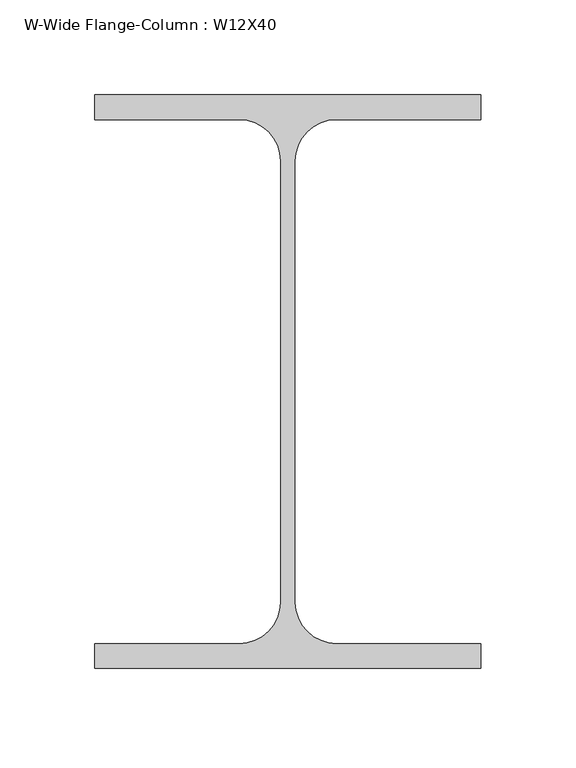
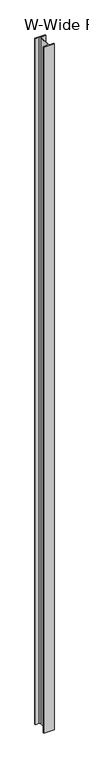
"""IFC4 building model written with IfcOpenShell, lengths in millimetres: column geometry, W-Wide Flange-Column : W12X40."""

from ifc_helpers import new_model, si_unit, point, frame, frame_2d, origin, place, context, project, spatial, polyline, circle_curve, trimmed, segment, composite_curve, outline, extrude, source, transform, mapped, element, save


def w_wide_flange_column_w12x40_26afb3f0(model_context):
    return source(origin(), model_context, "Body", "SweptSolid", [
        extrude(outline(composite_curve([segment(polyline([(101.727, 151.13), (101.727, 138.049), (25.5905, 138.049)]), True, "CONTINUOUS"), segment(trimmed(circle_curve(frame_2d((25.5905, 116.205)), 21.844), [point((25.5905, 138.049))], [point((3.7465, 116.205))], True, "CARTESIAN"), True, "CONTINUOUS"), segment(polyline([(3.7465, 116.205), (3.7465, -116.205)]), True, "CONTINUOUS"), segment(trimmed(circle_curve(frame_2d((25.5905, -116.205)), 21.844), [point((3.7465, -116.205))], [point((25.5905, -138.049))], True, "CARTESIAN"), True, "CONTINUOUS"), segment(polyline([(25.5905, -138.049), (101.727, -138.049), (101.727, -151.13), (-101.727, -151.13), (-101.727, -138.049), (-25.5905, -138.049)]), True, "CONTINUOUS"), segment(trimmed(circle_curve(frame_2d((-25.5905, -116.205)), 21.844), [point((-25.5905, -138.049))], [point((-3.7465, -116.205))], True, "CARTESIAN"), True, "CONTINUOUS"), segment(polyline([(-3.7465, -116.205), (-3.7465, 116.205)]), True, "CONTINUOUS"), segment(trimmed(circle_curve(frame_2d((-25.5905, 116.205)), 21.844), [point((-3.7465, 116.205))], [point((-25.5905, 138.049))], True, "CARTESIAN"), True, "CONTINUOUS"), segment(polyline([(-25.5905, 138.049), (-101.727, 138.049), (-101.727, 151.13), (101.727, 151.13)]), True, "CONTINUOUS")], self_intersect=False)), frame((0.0, 0.0, 17627.6), z_axis=(0.0, 0.0, 1.0), x_axis=(1.0, 0.0, 0.0)), (0.0, 0.0, 1.0), 14357.35),
    ])


if __name__ == "__main__":
    model = new_model("IFC4")
    model_context = context("Model", 3, world=origin())
    ifc_project = project(units=[si_unit("LENGTHUNIT", "METRE", prefix="MILLI")], contexts=[model_context])
    site = spatial("IfcSite", under=ifc_project)
    building = spatial("IfcBuilding", under=site)
    placement = place(None, origin())
    w_wide_flange_column_w12x40_shape = w_wide_flange_column_w12x40_26afb3f0(model_context)
    element("IfcColumn", 1, ObjectType="W-Wide Flange-Column : W12X40", at=placement, inside=building, context=model_context, shape_type="MappedRepresentation", body=[
        mapped(w_wide_flange_column_w12x40_shape, transform((0.0, 0.0, 0.0), x_axis=(1.0, 0.0, 0.0), y_axis=(0.0, 1.0, 0.0), z_axis=(0.0, 0.0, 1.0))),
    ])
    save(model, "model.ifc")

# Revit data of these elements
# Type "W-Wide Flange-Column : W12X40"
#   Assembly Code = "B10"
#   W = 40
#   bf = 0' - 8.01"
#   d = 0' - 11.9"
#   k = 0' - 1 3/8"
#   kr = 0' - 0.86"
#   tf = 0' - 0.515"
#   tw = 0' - 0.295"
#   A = 0.08125 SF
#   Structural Material [instance default] = Steel ASTM A992
# Element 1 (IfcColumn, "W-Wide Flange-Column : W12X40")
#   Materials on its faces: "Steel ASTM A992"
# Materials
#   "Steel ASTM A992": class "Metal", colour RGB 199 199 199, transparency 0, Description = "Structural steel 50ksi", Cost = 0
